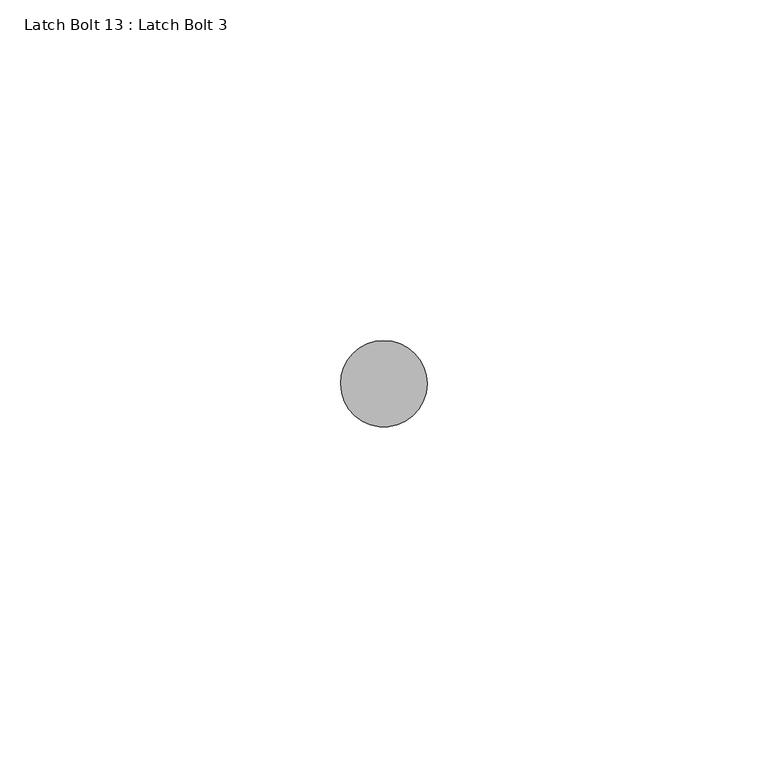
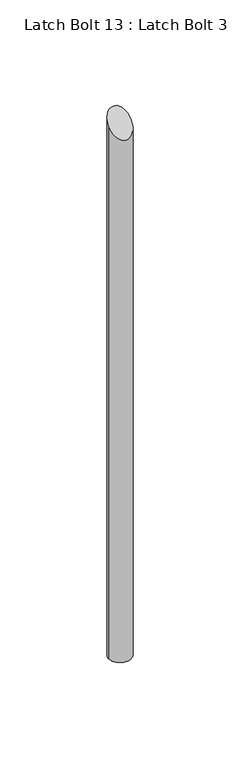
"""IFC4 building model written with IfcOpenShell, lengths in millimetres: proxy geometry, Latch Bolt 13 : Latch Bolt 3."""

from ifc_helpers import new_model, si_unit, frame, origin, place, context, project, spatial, circle_curve, ellipse_curve, source, transform, mapped, element, save
from ifc_brep_helpers import plane_surface, cylinder_surface, advanced_brep


def latch_bolt_13_latch_bolt_3_89fb1f9d(model_context):
    return source(origin(), model_context, "Body", "AdvancedBrep", [
        advanced_brep(
        [(587315.8935739, -535163.4663841, -25.4), (587303.1935739, -535163.4663841, -25.4), (587303.1935739, -535163.4663841, 292.0822144), (587309.5435739, -535157.1163841, 298.4322144), (587315.8935739, -535163.4663841, 292.0822144)],
        [
            (0, 1, circle_curve(frame((587309.5435739, -535163.4663841, -25.4), z_axis=(0.0, 0.0, -1.0), x_axis=(1.0, 0.0, 0.0)), 6.35)),
            (1, 0, circle_curve(frame((587309.5435739, -535163.4663841, -25.4), z_axis=(0.0, 0.0, -1.0), x_axis=(1.0, 0.0, 0.0)), 6.35)),
            (1, 2),
            (2, 3, ellipse_curve(frame((587309.5435739, -535163.4663841, 292.0822144), z_axis=(0.0, 0.7071067811865513, -0.7071067811865438), x_axis=(0.0, 0.7071067811865438, 0.7071067811865512)), 8.9802561, 6.35)),
            (3, 4, ellipse_curve(frame((587309.5435739, -535163.4663841, 292.0822144), z_axis=(0.0, 0.7071067811865513, -0.7071067811865438), x_axis=(0.0, 0.7071067811865438, 0.7071067811865512)), 8.9802561, 6.35)),
            (4, 0),
            (4, 2, ellipse_curve(frame((587309.5435739, -535163.4663841, 292.0822144), z_axis=(0.0, 0.7071067811865513, -0.7071067811865438), x_axis=(0.0, 0.7071067811865438, 0.7071067811865512)), 8.9802561, 6.35)),
        ],
        [
            plane_surface(frame((587315.8935739, -535163.4663841, -25.4), z_axis=(0.0, 0.0, -1.0), x_axis=(0.0, -1.0, 0.0))),
            cylinder_surface(frame((587309.5435739, -535163.4663841, -25.4), z_axis=(0.0, 0.0, 1.0), x_axis=(1.0, 0.0, 0.0)), 6.35),
            plane_surface(frame((587338.1185739, -535157.1163841, 298.4322144), z_axis=(0.0, -0.7071067811865513, 0.7071067811865438), x_axis=(-1.0, 0.0, 0.0))),
        ],
        [
            (0, [[1, 2]]),
            (1, [[-2, 3, 4, 5, 6]]),
            (1, [[-1, -6, 7, -3]]),
            (2, [[-5, -4, -7]]),
        ],
    ),
    ])


if __name__ == "__main__":
    model = new_model("IFC4")
    model_context = context("Model", 3, world=origin())
    ifc_project = project(units=[si_unit("LENGTHUNIT", "METRE", prefix="MILLI")], contexts=[model_context])
    site = spatial("IfcSite", under=ifc_project)
    building = spatial("IfcBuilding", under=site)
    placement = place(None, origin())
    latch_bolt_13_latch_bolt_3_shape = latch_bolt_13_latch_bolt_3_89fb1f9d(model_context)
    element("IfcBuildingElementProxy", 1, Name="Latch Bolt 13 : Latch Bolt 3", ObjectType="Latch Bolt 13 : Latch Bolt 3", at=placement, inside=building, context=model_context, shape_type="MappedRepresentation", body=[
        mapped(latch_bolt_13_latch_bolt_3_shape, transform((0.0, 0.0, 0.0), x_axis=(1.0, 0.0, 0.0), y_axis=(0.0, 1.0, 0.0), z_axis=(0.0, 0.0, 1.0))),
    ])
    save(model, "model.ifc")

# Revit data of these elements
# Element 1 (IfcBuildingElementProxy, "Latch Bolt 13 : Latch Bolt 3")
#   Materials on its faces: "GALV. SLIDE BOLT"
# Materials
#   "GALV. SLIDE BOLT": class "Metal", colour RGB 189 187 185, transparency 0, Description = "Carbon steel", Cost = 0
